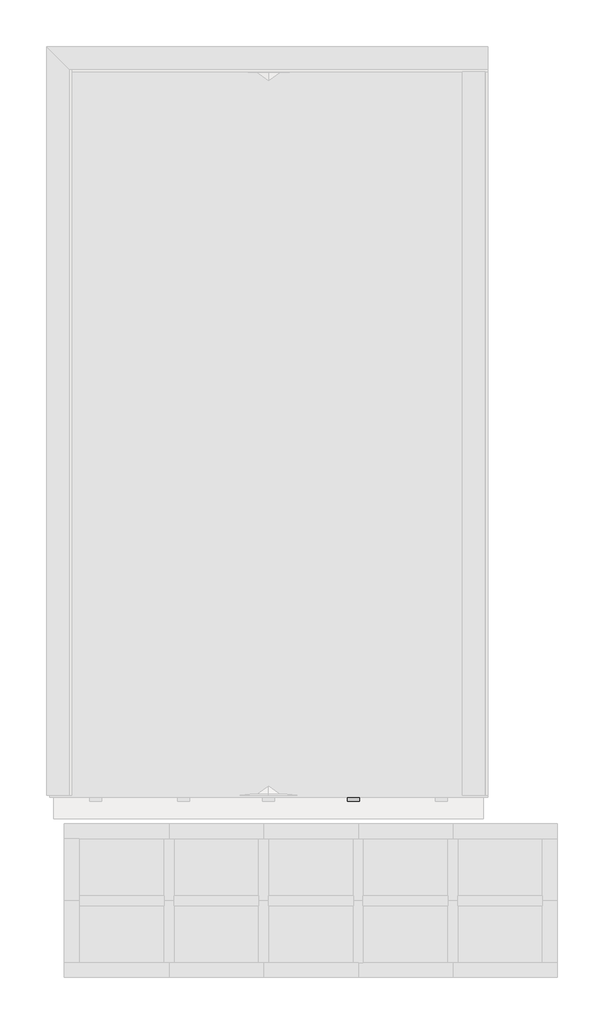
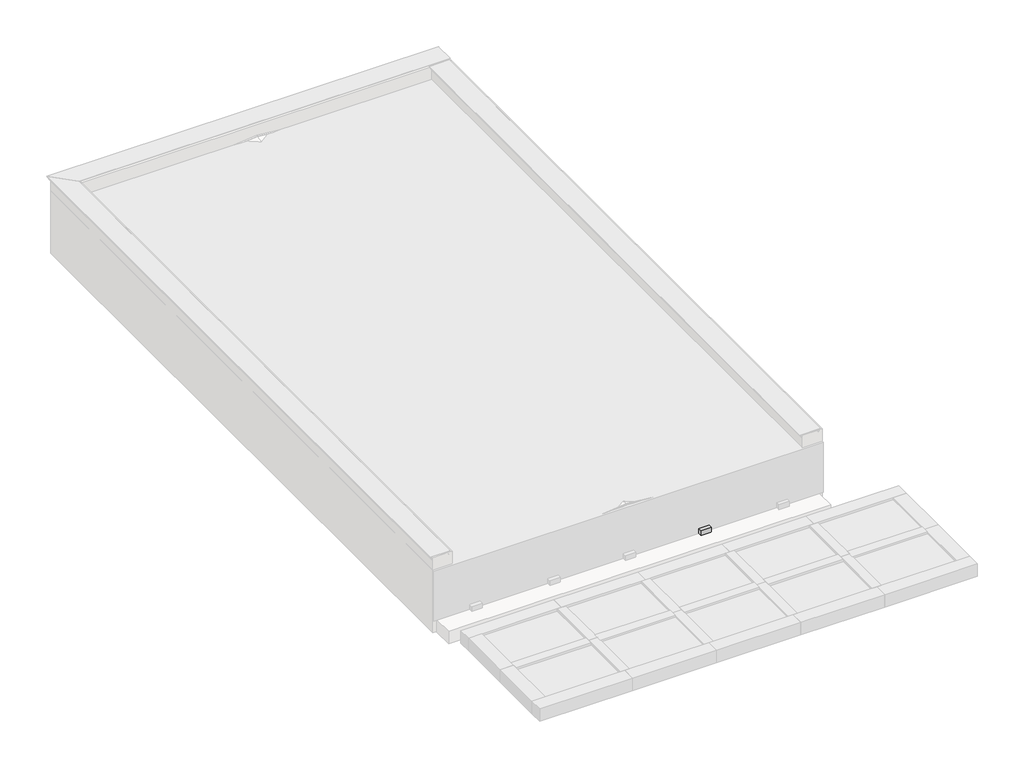
# One storey, part 2 of 3: 38 beams, 6 columns.
# Revit data of these elements (continued)
# Type "Madeira de lei : Berço 6x12cm"
#   A = 0.02 m²
#   Length [instance default] = 1.524 m
#   b = 0.06 m
#   d = 0.12 m
#   Structural Material [instance default] = none
#   Assembly Code = ""
# Type "Cumeeira Telha Ondulada : Fibrocimento"
#   Cost = 5
#   Length [instance default] = 1.524 m
#   b = 0.07 m
#   h = 0.16 m
#   Structural Material = .TELHA DE FIBROCIMENTO
#   Assembly Code = ""
# Type "Telha Ondulada : Fibrocimento"
#   Description = "TELHA ONDULADA FIBROCIMENTO"
#   Cost = 5
#   Length [instance default] = 1.524 m
#   b = 0.07 m
#   h = 0.16 m
#   Structural Material = .TELHA DE FIBROCIMENTO
#   Assembly Code = ""
# Type "Madeira de lei : Viga Cumeeira 6x16cm"
#   A = 0.02 m²
#   Length [instance default] = 1.524 m
#   b = 0.06 m
#   d = 0.16 m
#   Structural Material [instance default] = none
#   Assembly Code = ""
# Type "Madeira de lei-Coluna : Pontalete 6X16cm"
#   A = 0.01952 m²
#   b = 0.06 m
#   d = 0.16 m
#   Structural Material [instance default] = none
#   Assembly Code = ""
# Elements 1, 2, 3, 4, 6, 7 (IfcBeam, "Madeira de lei : Berço 6x12cm")
#   Comments = ""
#   Uso = "TELHADOS ESTRUTURAS"
#   Compr Cmcl = 6.00 m
#   Structural Material = .MADEIRAMENTO
#   Phase Created = CC_AP
#   Materials on its faces: ".MADEIRAMENTO"
# Element 5 (IfcBeam, "Madeira de lei : Berço 6x12cm")
#   Comments = ""
#   Uso = "TELHADOS ESTRUTURAS"
#   Compr Cmcl = 7.00 m
#   Structural Material = .MADEIRAMENTO
#   Phase Created = CC_AP
#   Materials on its faces: ".MADEIRAMENTO"
# Element 8 (IfcBeam, "Cumeeira Telha Ondulada : Fibrocimento")
#   Comments = ""
#   Uso = "TELHADOS TELHAS"
#   Phase Created = CC_AP
#   Materials on its faces: ".TELHA DE FIBROCIMENTO"
# Elements 9, 10, 11, 12, 13, 14, 15, 16, 17, 18, 19, 20, 21, 22, 23, 24, 25, 26, 27, 28, 29, 30, 31, 32, 33, 34, 35, 36, 37 (IfcBeam, "Telha Ondulada : Fibrocimento")
#   Uso = "TELHADOS TELHAS"
#   Phase Created = CC_AP
#   Materials on its faces: ".TELHA DE FIBROCIMENTO"
# Element 38 (IfcBeam, "Madeira de lei : Viga Cumeeira 6x16cm")
#   Comments = ""
#   Uso = "TELHADOS MADEIRAMENTO"
#   Compr Cmcl = 7.50 m
#   Structural Material = .MADEIRAMENTO
#   Phase Created = CC_AP
#   Materials on its faces: ".MADEIRAMENTO"
# Elements 39, 40, 41, 42, 43, 44 (IfcColumn, "Madeira de lei-Coluna : Pontalete 6X16cm")
#   Comments = ""
#   Uso = "TELHADOS ESTRUTURAS"
#   Compr Cmcl = 2.00 m
#   Structural Material = .MADEIRAMENTO
#   Phase Created = CC_AP
#   Materials on its faces: ".MADEIRAMENTO"
# Materials
#   ".TELHA DE FIBROCIMENTO": class "CC_TELHADO", colour RGB 77 77 76, transparency 0, Description = "TELHA ONDULADA FIBROCIMENTO", Cost = 0
#   ".MADEIRAMENTO": class ".CC_MADEIRAS", colour RGB 212 179 113, transparency 0, Cost = 0
# Room, not placed, phase "CC_AP", upper offset 0.00 m, lower offset 0.00 m
#   Number = "31"
#   Name = "Room"
# Room, not placed, phase "CC_AP", upper offset 0.00 m, lower offset 0.00 m
#   Number = "34"
#   Name = "Room"
